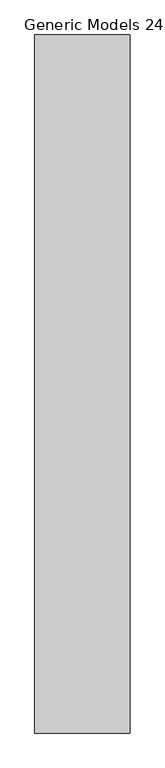
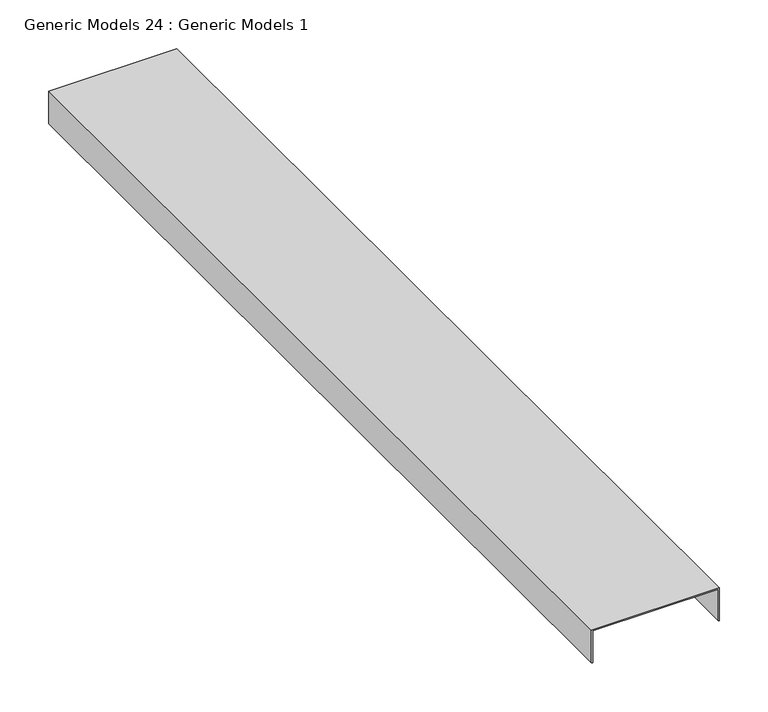
"""IFC4 building model written with IfcOpenShell, lengths in millimetres: proxy geometry, Generic Models 24 : Generic Models 1."""

from ifc_helpers import new_model, si_unit, frame, origin, place, context, project, spatial, polyline, outline, extrude, source, transform, mapped, element, save


def generic_models_24_generic_models_1_cb36caf6(model_context):
    return source(origin(), model_context, "Body", "SweptSolid", [
        extrude(outline(polyline([(2826.0822008, 55668.3562571), (2784.8072008, 55668.3562571), (2784.8072008, 55669.9437571), (2824.4947008, 55669.9437571), (2824.4947008, 55819.1687571), (2784.8072008, 55819.1687571), (2784.8072008, 55820.7562571), (2826.0822008, 55820.7562571), (2826.0822008, 55668.3562571)])), frame((0.0, 36117.4598594, 0.0), z_axis=(0.0, 1.0, 0.0), x_axis=(0.0, 0.0, 1.0)), (0.0, 0.0, 1.0), 1117.6),
    ])


if __name__ == "__main__":
    model = new_model("IFC4")
    model_context = context("Model", 3, world=origin())
    ifc_project = project(units=[si_unit("LENGTHUNIT", "METRE", prefix="MILLI")], contexts=[model_context])
    site = spatial("IfcSite", under=ifc_project)
    building = spatial("IfcBuilding", under=site)
    placement = place(None, origin())
    generic_models_24_generic_models_1_shape = generic_models_24_generic_models_1_cb36caf6(model_context)
    element("IfcBuildingElementProxy", 1, Name="Generic Models 24 : Generic Models 1", ObjectType="Generic Models 24 : Generic Models 1", at=placement, inside=building, context=model_context, shape_type="MappedRepresentation", body=[
        mapped(generic_models_24_generic_models_1_shape, transform((0.0, 0.0, 0.0), x_axis=(1.0, 0.0, 0.0), y_axis=(0.0, 1.0, 0.0), z_axis=(0.0, 0.0, 1.0))),
    ])
    save(model, "model.ifc")

# Revit data of these elements
# Element 1 (IfcBuildingElementProxy, "Generic Models 24 : Generic Models 1")
#   Materials on its faces: "METAL STUDS"
# Materials
#   "METAL STUDS": class "Unassigned", colour RGB 210 209 208, transparency 0, Keynote = "M05121300.02", Cost = 0
